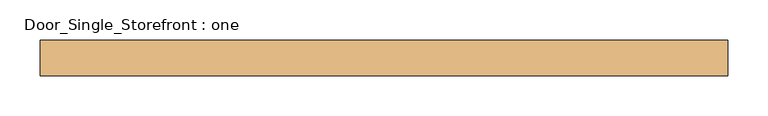
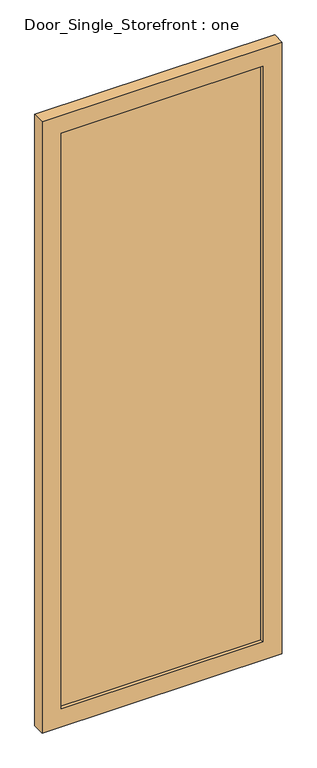
"""IFC4 building model written with IfcOpenShell, lengths in millimetres: door geometry, Door_Single_Storefront : one."""

from ifc_helpers import new_model, si_unit, frame, origin, place, context, project, spatial, polyline, outline, extrude, source, transform, mapped, element, save


def door_single_storefront_one_247823ef(model_context):
    return source(origin(), model_context, "Body", "SweptSolid", [
        extrude(outline(polyline([(361.2994325, 6.35), (361.2994325, -12.7), (-361.2994325, -12.7), (-361.2994325, 6.35), (361.2994325, 6.35)])), frame((0.0, 0.0, 68.2625), z_axis=(0.0, 0.0, 1.0), x_axis=(1.0, 0.0, 0.0)), (0.0, 0.0, 1.0), 2176.3830968),
        extrude(outline(polyline([(2312.9080968, -429.5619325), (0.0, -429.5619325), (0.0, 429.5619325), (2312.9080968, 429.5619325), (2312.9080968, -429.5619325)]), holes=[polyline([(68.2625, 361.2994325), (68.2625, -361.2994325), (2244.6455968, -361.2994325), (2244.6455968, 361.2994325), (68.2625, 361.2994325)])]), frame((0.0, -25.4, 0.0), z_axis=(0.0, 1.0, 0.0), x_axis=(0.0, 0.0, 1.0)), (0.0, 0.0, 1.0), 44.45),
    ])


if __name__ == "__main__":
    model = new_model("IFC4")
    model_context = context("Model", 3, world=origin())
    ifc_project = project(units=[si_unit("LENGTHUNIT", "METRE", prefix="MILLI")], contexts=[model_context])
    site = spatial("IfcSite", under=ifc_project)
    building = spatial("IfcBuilding", under=site)
    placement = place(None, origin())
    door_single_storefront_one_shape = door_single_storefront_one_247823ef(model_context)
    element("IfcDoor", 1, ObjectType="Door_Single_Storefront : one", at=placement, inside=building, context=model_context, shape_type="MappedRepresentation", body=[
        mapped(door_single_storefront_one_shape, transform((0.0, 0.0, 0.0), x_axis=(1.0, 0.0, 0.0), y_axis=(0.0, 1.0, 0.0), z_axis=(0.0, 0.0, 1.0))),
    ])
    save(model, "model.ifc")

# Revit data of these elements
# Type "Door_Single_Storefront : one"
#   Type Mark = "29"
#   OD_DS_Door_Material = "ALUM./GLAZING"
#   OD_DS_Door_Type = "STOREFRONT (NARROW STILE)"
#   OD_DS_Lockset = "ENTRY LOCK (INSIDE ADA LEVER ALWAYS ACTIVE)"
#   Analytic Construction = "<None>"
#   angle open [instance default] = 132.952°
#   Stile_Width = 0' - 2 11/16"
#   Door_Thickness = 0' - 1 3/4"
#   Door_Offset = 0' - 1"
#   Glass_Material = TEMPERED INSULATED GLAZING (CARDINAL GLASS LoĒ²-240\nOR EQUIVALENT)
#   Frame_Material = KAWNEER 260 INSULCLADTM THERMAL ENTRANCE - CLEAR ANODIZED ALUM.
#   Function = (empty or 0)
# Element 1 (IfcDoor, "Door_Single_Storefront : one")
#   angle open = 170.00°
#   Materials on its faces: "KAWNEER 260 INSULCLADTM THERMAL ENTRANCE - CLEAR ANODIZED ALUM.", "TEMPERED INSULATED GLAZING (CARDINAL GLASS LoĒ²-240\nOR EQUIVALENT)"
# Materials
#   "TEMPERED INSULATED GLAZING (CARDINAL GLASS LoĒ²-240\nOR EQUIVALENT)": class "Glass", colour RGB 196 205 210, transparency 0.85, Description = "Soda Lime Glass", Cost = 0
#   "KAWNEER 260 INSULCLADTM THERMAL ENTRANCE - CLEAR ANODIZED ALUM.": class "Metal", colour RGB 244 244 244, transparency 0, Description = "Aluminum 6061", Cost = 0
